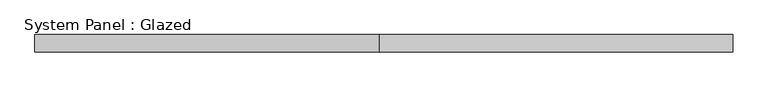
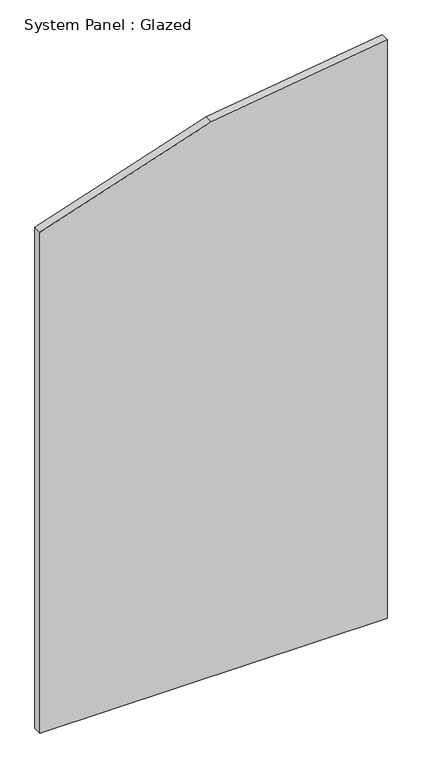
"""IFC4 building model written with IfcOpenShell, lengths in millimetres: plate geometry, System Panel : Glazed."""

from ifc_helpers import new_model, si_unit, frame, origin, place, context, project, spatial, polyline, outline, extrude, source, transform, mapped, element, save


def system_panel_glazed_6c4c7ed2(model_context):
    return source(origin(), model_context, "Body", "SweptSolid", [
        extrude(outline(polyline([(0.0, -500.0), (0.0, 500.0), (1761.3177476, 500.0), (1689.3102197, -6.2307384), (1526.050305, -500.0), (0.0, -500.0)])), frame((0.0, 24.5, 0.0), z_axis=(0.0, 1.0, 0.0), x_axis=(0.0, 0.0, 1.0)), (0.0, 0.0, 1.0), 25.0),
    ])


if __name__ == "__main__":
    model = new_model("IFC4")
    model_context = context("Model", 3, world=origin())
    ifc_project = project(units=[si_unit("LENGTHUNIT", "METRE", prefix="MILLI")], contexts=[model_context])
    site = spatial("IfcSite", under=ifc_project)
    building = spatial("IfcBuilding", under=site)
    placement = place(None, origin())
    system_panel_glazed_shape = system_panel_glazed_6c4c7ed2(model_context)
    element("IfcPlate", 1, ObjectType="System Panel : Glazed", at=placement, inside=building, context=model_context, shape_type="MappedRepresentation", body=[
        mapped(system_panel_glazed_shape, transform((0.0, 0.0, 0.0), x_axis=(1.0, 0.0, 0.0), y_axis=(0.0, 1.0, 0.0), z_axis=(0.0, 0.0, 1.0))),
    ])
    save(model, "model.ifc")

# Revit data of these elements
# Element 1 (IfcPlate, "System Panel : Glazed")
#   Materials on its faces: "Glass"
# Materials
#   "Glass": class "Glass", colour RGB 218 227 224, transparency 0.85, Description = "Soda Lime Glass", Cost = 0
